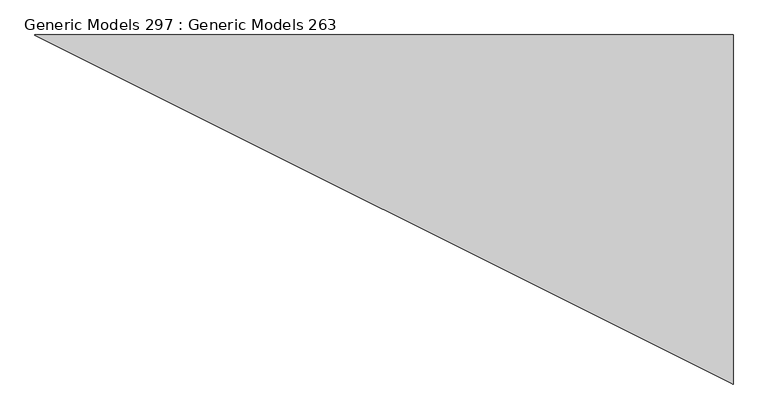
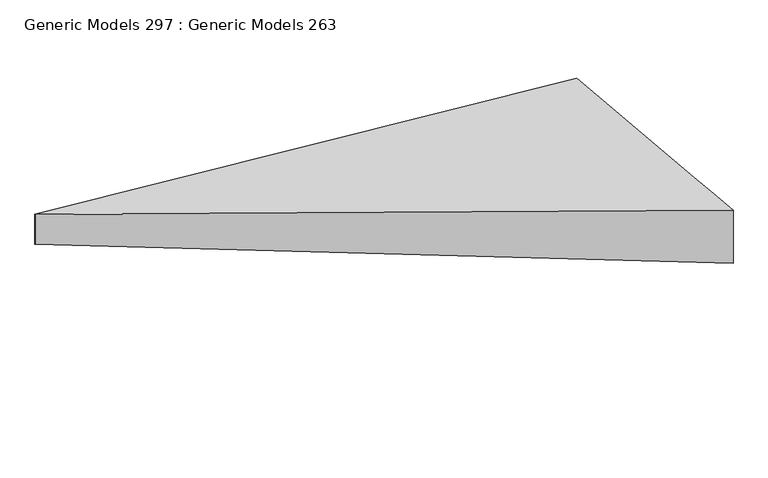
"""IFC4 building model written with IfcOpenShell, lengths in millimetres: proxy geometry, Generic Models 297 : Generic Models 263."""

from ifc_helpers import new_model, si_unit, frame, origin, place, context, project, spatial, source, transform, mapped, element, save
from ifc_brep_helpers import plane_surface, spline_surface, advanced_brep


def generic_models_297_generic_models_263_bc1a45ca(model_context):
    return source(origin(), model_context, "Body", "AdvancedBrep", [
        advanced_brep(
        [(91554.5797726, -8256.6272578, 2.0699085), (91554.5797726, -8256.6272578, -314.8198762), (91554.5797726, -6732.6272578, -314.8198762), (91554.5797726, -6732.6272578, -137.0198762), (88506.5797726, -6733.7737439, 120.3150753), (88506.5797726, -6732.6272578, 120.3150753), (88506.5797726, -6732.6272578, -58.1173502), (88506.5797726, -6733.7737439, -58.1173502)],
        [
            (0, 1),
            (1, 2),
            (2, 3),
            (3, 0),
            (4, 5),
            (5, 6),
            (6, 7),
            (7, 4),
            (7, 1),
            (0, 4),
            (6, 2),
            (5, 3),
        ],
        [
            plane_surface(frame((91554.5797726, -7494.6272578, -191.14743), z_axis=(1.0, 0.0, 0.0), x_axis=(0.0, 0.0, -1.0))),
            plane_surface(frame((88506.5797726, -6733.2005009, 31.0988625), z_axis=(-1.0, 0.0, 0.0), x_axis=(0.0, 0.0, -1.0))),
            plane_surface(frame((88506.5797726, -6733.7737439, 31.0988625), z_axis=(-0.4469443881993885, -0.894561744016071, 0.0), x_axis=(0.0, 0.0, -1.0))),
            plane_surface(frame((88506.5797726, -6733.2005009, -58.1173502), z_axis=(-0.08392288197547094, 0.0, -0.9964722524390387), x_axis=(0.0, 1.0, 0.0))),
            plane_surface(frame((88506.5797726, -6732.6272578, 31.0988625), z_axis=(0.0, 1.0, 0.0), x_axis=(0.0, 0.0, 1.0))),
            spline_surface(1, 1, [[(88506.5797726, -6732.6272578, 120.3150753), (91554.5797726, -6732.6272578, -137.0198762)], [(88506.5797726, -6733.7737439, 120.3150753), (91554.5797726, -8256.6272578, 2.0699085)]], [2, 2], [2, 2], [0.0, 1.0], [0.0, 1.0]),
        ],
        [
            (0, [[1, 2, 3, 4]]),
            (1, [[5, 6, 7, 8]]),
            (2, [[-8, 9, -1, 10]]),
            (3, [[-7, 11, -2, -9]]),
            (4, [[-6, 12, -3, -11]]),
            (5, [[-5, -10, -4, -12]]),
        ],
    ),
    ])


if __name__ == "__main__":
    model = new_model("IFC4")
    model_context = context("Model", 3, world=origin())
    ifc_project = project(units=[si_unit("LENGTHUNIT", "METRE", prefix="MILLI")], contexts=[model_context])
    site = spatial("IfcSite", under=ifc_project)
    building = spatial("IfcBuilding", under=site)
    placement = place(None, origin())
    generic_models_297_generic_models_263_shape = generic_models_297_generic_models_263_bc1a45ca(model_context)
    element("IfcBuildingElementProxy", 1, Name="Generic Models 297 : Generic Models 263", ObjectType="Generic Models 297 : Generic Models 263", at=placement, inside=building, context=model_context, shape_type="MappedRepresentation", body=[
        mapped(generic_models_297_generic_models_263_shape, transform((0.0, 0.0, 0.0), x_axis=(1.0, 0.0, 0.0), y_axis=(0.0, 1.0, 0.0), z_axis=(0.0, 0.0, 1.0))),
    ])
    save(model, "model.ifc")

# Revit data of these elements
# Element 1 (IfcBuildingElementProxy, "Generic Models 297 : Generic Models 263")
#   Materials on its faces: "SLOPED - 7\" CONC."
# Materials
#   "SLOPED - 7\" CONC.": class "Concrete", colour RGB 191 191 191, transparency 0, Description = "Cast-in-place concrete", Cost = 0
